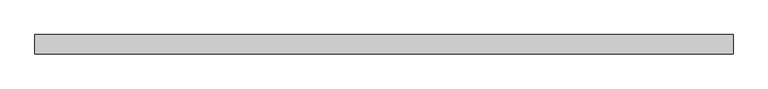
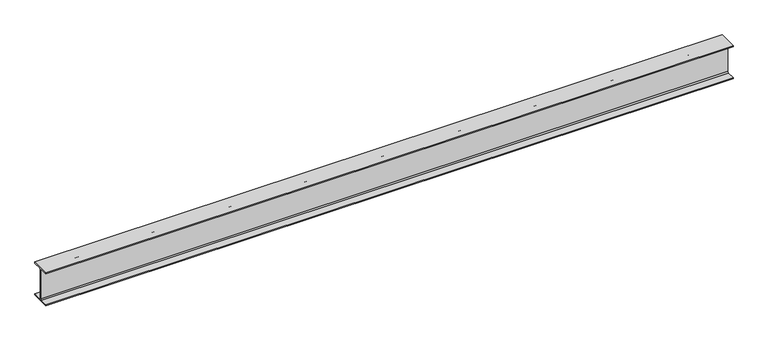
"""IFC4 building model written with IfcOpenShell, lengths in millimetres: beam geometry, Old_Steel Beam_H-KSD3502 : H_SB_ASB_H-390×300x10x16."""

from ifc_helpers import new_model, si_unit, point, frame, frame_2d, origin, place, context, project, spatial, polyline, circle_curve, trimmed, segment, composite_curve, outline, extrude, source, transform, mapped, element, save


def beam_73eeb3b6(model_context):
    return source(origin(), model_context, "Body", "SweptSolid", [
        extrude(outline(composite_curve([segment(polyline([(82.5, -141.5), (82.5, -151.7), (-82.5, -151.7), (-82.5, -141.5), (-11.9, -141.5)]), True, "CONTINUOUS"), segment(trimmed(circle_curve(frame_2d((-11.9, -132.6)), 8.9), [point((-11.9, -141.5))], [point((-3.0, -132.6))], True, "CARTESIAN"), True, "CONTINUOUS"), segment(polyline([(-3.0, -132.6), (-3.0, 132.6)]), True, "CONTINUOUS"), segment(trimmed(circle_curve(frame_2d((-11.9, 132.6)), 8.9), [point((-3.0, 132.6))], [point((-11.9, 141.5))], True, "CARTESIAN"), True, "CONTINUOUS"), segment(polyline([(-11.9, 141.5), (-82.5, 141.5), (-82.5, 151.7), (82.5, 151.7), (82.5, 141.5), (11.9, 141.5)]), True, "CONTINUOUS"), segment(trimmed(circle_curve(frame_2d((11.9, 132.6)), 8.9), [point((11.9, 141.5))], [point((3.0, 132.6))], True, "CARTESIAN"), True, "CONTINUOUS"), segment(polyline([(3.0, 132.6), (3.0, -132.6)]), True, "CONTINUOUS"), segment(trimmed(circle_curve(frame_2d((11.9, -132.6)), 8.9), [point((3.0, -132.6))], [point((11.9, -141.5))], True, "CARTESIAN"), True, "CONTINUOUS"), segment(polyline([(11.9, -141.5), (82.5, -141.5)]), True, "CONTINUOUS")], self_intersect=False)), frame((-2987.2999994, 0.0, 0.0), z_axis=(1.0, 0.0, 0.0), x_axis=(0.0, 1.0, 0.0)), (0.0, 0.0, 1.0), 5974.5999988),
    ])


if __name__ == "__main__":
    model = new_model("IFC4")
    model_context = context("Model", 3, world=origin())
    ifc_project = project(units=[si_unit("LENGTHUNIT", "METRE", prefix="MILLI")], contexts=[model_context])
    site = spatial("IfcSite", under=ifc_project)
    building = spatial("IfcBuilding", under=site)
    placement = place(None, origin())
    beam_shape = beam_73eeb3b6(model_context)
    element("IfcBeam", 1, ObjectType="Old_Steel Beam_H-KSD3502 : H_SB_ASB_H-390×300x10x16", at=placement, inside=building, context=model_context, shape_type="MappedRepresentation", body=[
        mapped(beam_shape, transform((0.0, 0.0, 0.0), x_axis=(1.0, 0.0, 0.0), y_axis=(0.0, 1.0, 0.0), z_axis=(0.0, 0.0, 1.0))),
    ])
    save(model, "model.ifc")

# Revit data of these elements
# Type "Old_Steel Beam_H-KSD3502 : H_SB_ASB_H-390×300x10x16"
#   Width = 30.0 cm
#   Web Thickness = 1.0 cm
#   Web Fillet = 2.2 cm
#   Warping Constant = 2517770.0 cm⁶
#   Torsional Moment of Inertia = 94.3867 cm⁴
#   Torsional Modulus = 1.0 cm³
#   Section Area = 136.0 cm²
#   Plastic Modulus weak axis = 733.0 cm³
#   Plastic Modulus strong axis = 2190.0 cm³
#   Perimeter = 1.92 m²/m
#   Nominal Weight = 107.00 kgf/m
#   Moment of Inertia weak axis = 7210.00 cm⁴
#   Moment of Inertia strong axis = 38700.00 cm⁴
#   Height = 39.0 cm
#   Flange Thickness = 1.6 cm
#   Elastic Modulus weak axis = 481.0 cm³
#   Elastic Modulus strong axis = 1980.0 cm³
#   Centroid Vertical = 19.5 cm
#   Centroid Horizontal = 15.0 cm
#   Length [instance default] = 1.5240 m
#   Structural Material [instance default] = Steel, 45-345
#   Assembly Code = ""
# Element 1 (IfcBeam, "Old_Steel Beam_H-KSD3502 : H_SB_ASB_H-390×300x10x16")
#   Structural Material = none
# Materials
#   "Steel, 45-345": class "Metal", colour RGB 189 187 185, transparency 0, Description = "Steel 345 MPa", Cost = 0
